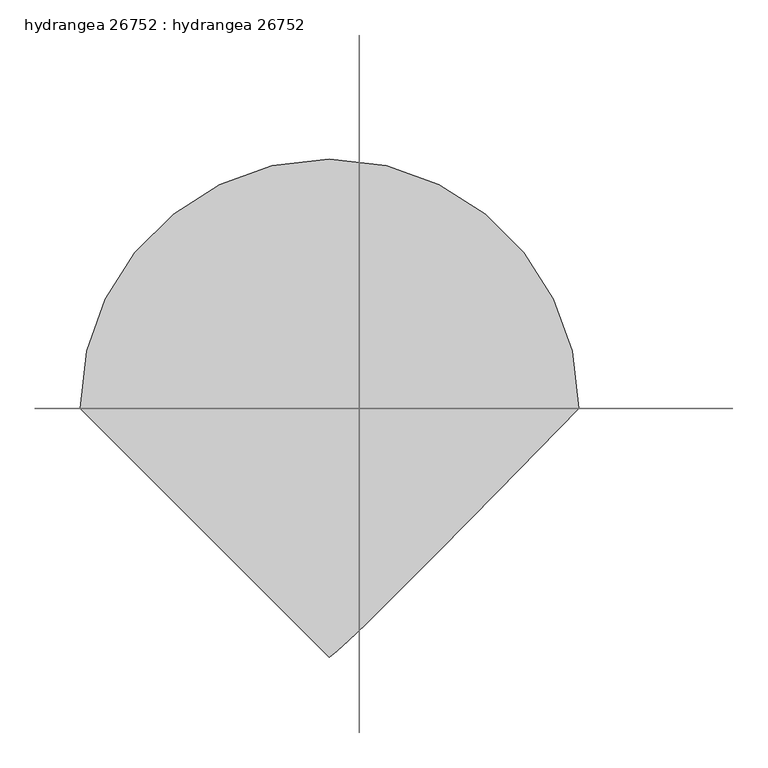
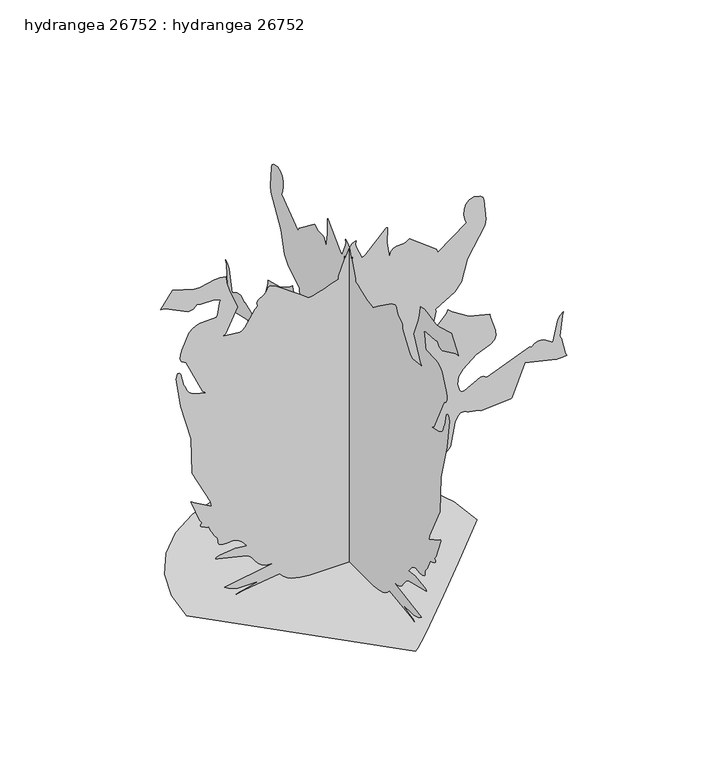
"""IFC4 building model written with IfcOpenShell, lengths in millimetres: proxy geometry, hydrangea 26752 : hydrangea 26752."""

from ifc_helpers import new_model, si_unit, origin, place, context, project, spatial, triangles, source, transform, mapped, element, save


def hydrangea_26752_hydrangea_26752_06a88d80(model_context):
    return source(origin(), model_context, "Body", "Tessellation", [
        triangles([(-464.7672343, 0.0, 3.02e-05), (-452.4787039, 106.4936905, 3.02e-05), (-417.4875984, 204.2914365, 3.02e-05), (-362.5905132, 290.5916013, 3.02e-05), (-290.5916013, 362.5905132, 3.02e-05), (-204.2911822, 417.4875984, 3.02e-05), (-106.4936905, 452.4787039, 3.02e-05), (2.03e-05, 464.7672343, 3.02e-05), (106.4939449, 452.4787039, 3.02e-05), (204.2914365, 417.4875984, 3.02e-05), (290.5916013, 362.5905132, 3.02e-05), (362.5905132, 290.5916013, 3.02e-05), (417.4875984, 204.2911822, 3.02e-05), (452.4787039, 106.4936905, 3.02e-05), (464.7672343, -4.06e-05, 3.02e-05), (313.7284884, -154.9290062, 3.02e-05), (201.7549816, -268.9964805, 3.02e-05), (122.337727, -349.0116546, 3.02e-05), (68.9646404, -401.7878663, 3.02e-05), (35.1246865, -434.1297149, 3.02e-05), (14.3067201, -452.8546257, 3.02e-05), (-6.09e-05, -464.7672343, 3.02e-05), (56.0289111, 377.7746518, 894.66276), (56.0289111, 434.8662978, 988.0256659), (56.0289111, 437.025323, 1007.8783058), (56.0289111, 431.6938534, 1074.0784075), (56.0289111, 427.5688871, 1084.5381615), (56.0289111, 420.2181004, 1091.4545998), (56.0289111, 399.2732306, 1096.0341894), (56.0289111, 384.089092, 1091.3859993), (56.0289111, 374.1170626, 1079.9991943), (56.0289111, 368.8109911, 1064.3553091), (56.0289111, 367.6197121, 1046.9435812), (56.0289111, 369.9971832, 1030.2455452), (56.0289111, 375.3946735, 1016.7479679), (56.0289111, 283.8809099, 949.5141357), (56.0289111, 278.4503729, 960.8348837), (56.0289111, 192.0161139, 1027.487138), (56.0289111, 183.512436, 1019.3997683), (56.0289111, 173.3158381, 1016.575304), (56.0289111, 151.4921339, 1016.077442), (56.0289111, 141.6905156, 1013.0776978), (56.0289111, 133.8441922, 1004.6956512), (56.0289111, 128.8665527, 988.2669302), (56.0289111, 120.2805761, 1038.0128763), (56.0289111, 121.9587531, 1087.6699471), (56.0289111, 121.3283319, 1088.8815737), (56.0289111, 120.3204537, 1089.2625824), (56.0289111, 119.0941387, 1088.975536), (56.0289111, 117.8101691, 1088.1856133), (56.0289111, 51.0174846, 1022.5290831), (56.0289111, 40.1538944, 1015.3484894), (56.0289111, 21.3923125, 1059.6105406), (56.0289111, 19.9031842, 1068.9729778), (56.0289111, 20.5441289, 1080.248089), (56.0289111, 9.1964113, 1074.4568727), (56.0289111, 0.5405762, 1063.7304199), (56.0289111, -13.2029357, 1031.7950146), (56.0289111, -15.0194446, 1031.1828426), (56.0289111, -16.1084712, 1040.5605406), (56.0289111, -15.8290449, 1030.10333), (56.0289111, -34.9326629, 980.1719301), (56.0289111, -34.6535171, 969.7147923), (56.0289111, -46.9016657, 965.6583538), (56.0289111, -59.853396, 960.979715), (56.0289111, -73.3885619, 956.0013124), (56.0289111, -87.3888065, 951.0482718), (56.0289111, -101.7342336, 946.4457911), (56.0289111, -116.3062366, 942.5138363), (56.0289111, -130.9854187, 939.5776056), (56.0289111, -158.8299491, 961.2921232), (56.0289111, -234.3038488, 1015.5618484), (56.0289111, -252.5433605, 1023.7431805), (56.0289111, -260.6957517, 1020.4259411), (56.0289111, -264.4829115, 1008.7952557), (56.0289111, -270.9573709, 1001.4368385), (56.0289111, -292.1841821, 987.7081707), (56.0289111, -295.084859, 980.1414814), (56.0289111, -293.5100641, 968.1907574), (56.0289111, -301.5567932, 960.9593674), (56.0289111, -333.5786213, 911.8103325), (56.0289111, -341.9555446, 903.575588), (56.0289111, -350.6474195, 900.6063652), (56.0289111, -405.2778059, 906.5576008), (56.0289111, -397.091387, 912.3182957), (56.0289111, -357.3022459, 989.5521715), (56.0289111, -383.3829941, 1051.2462982), (56.0289111, -392.869915, 1083.2706516), (56.0289111, -394.0713315, 1102.6610378), (56.0289111, -413.8020676, 1107.4693199), (56.0289111, -431.2518745, 1106.8977705), (56.0289111, -479.0928497, 1096.097703), (56.0289111, -496.5959965, 1097.2025774), (56.0289111, -565.8923844, 1117.6013323), (56.0289111, -605.1150993, 1065.3077946), (56.0289111, -590.4389603, 1063.2046526), (56.0289111, -515.963528, 1028.2542423), (56.0289111, -499.8980115, 1030.0398165), (56.0289111, -487.4520052, 1042.8973166), (56.0289111, -476.9008324, 1039.305748), (56.0289111, -431.2823596, 1037.8351255), (56.0289111, -421.2823886, 1035.6633831), (56.0289111, -412.7479531, 1030.7561245), (56.0289111, -416.4106656, 1023.8879391), (56.0289111, -422.1561361, 984.398489), (56.0289111, -425.8213557, 977.5278328), (56.0289111, -478.1860737, 974.7465345), (56.0289111, -490.5939646, 971.7493338), (56.0289111, -502.2144762, 965.7473019), (56.0289111, -512.7834532, 955.7015488), (56.0289111, -536.4029417, 906.3493286), (56.0289111, -540.7590348, 890.4260273), (56.0289111, -541.4473649, 876.4001392), (56.0289111, -536.9465132, 865.9378418), (56.0289111, -523.4413055, 857.3729576), (56.0289111, -470.3247439, 742.9737631), (56.0289111, -459.1462111, 734.3275612), (56.0289111, -495.4784048, 743.0092987), (56.0289111, -506.2683349, 747.8099504), (56.0289111, -515.3336246, 754.7263887), (56.0289111, -522.0366674, 764.454574), (56.0289111, -525.7400024, 777.6930828), (56.0289111, -531.1476665, 784.7339321), (56.0289111, -539.8243172, 825.0565435), (56.0289111, -543.8298866, 829.879941), (56.0289111, -550.6015663, 829.2856459), (56.0289111, -555.6434461, 813.3064613), (56.0289111, -540.8123746, 716.5628025), (56.0289111, -507.4392663, 594.6655191), (56.0289111, -503.093347, 475.8365441), (56.0289111, -444.0484045, 359.0446904), (56.0289111, -441.1045435, 344.0002235), (56.0289111, -497.2995872, 374.7622267), (56.0289111, -506.1286268, 381.752316), (56.0289111, -507.3122755, 379.8777938), (56.0289111, -479.3442879, 309.3622215), (56.0289111, -471.5769931, 298.1760402), (56.0289111, -476.8474926, 293.4109968), (56.0289111, -476.8347754, 288.7729441), (56.0289111, -473.0577893, 284.5159002), (56.0289111, -460.289201, 278.1963731), (56.0289111, -454.3303714, 276.6495199), (56.0289111, -450.6829196, 276.5250544), (56.0289111, -447.9727289, 270.8405358), (56.0289111, -445.4428688, 265.374445), (56.0289111, -442.9105016, 259.9769365), (56.0289111, -440.1901734, 254.4981467), (56.0289111, -437.1015175, 248.789756), (56.0289111, -433.4642395, 242.6990667), (56.0289111, -429.0903422, 236.0780501), (56.0289111, -423.9341526, 231.4173971), (56.0289111, -421.2519035, 226.5421133), (56.0289111, -420.2282742, 221.6594716), (56.0289111, -420.0530305, 216.9764544), (56.0289111, -419.910779, 212.7001166), (56.0289111, -418.9912857, 209.0374223), (56.0289111, -416.4817732, 206.1956808), (56.0289111, -404.3481751, 201.1304013), (56.0289111, -392.979138, 200.8065475), (56.0289111, -381.7802576, 202.325223), (56.0289111, -370.1622894, 202.7872406), (56.0289111, -357.5257424, 199.293722), (56.0289111, -343.2814084, 188.9454982), (56.0289111, -326.8374267, 168.843146), (56.0289111, -363.7335394, 174.8182537), (56.0289111, -415.2447847, 168.959745), (56.0289111, -424.7621907, 165.1799612), (56.0289111, -427.6882476, 161.3724901), (56.0289111, -422.6031655, 158.3819023), (56.0289111, -326.8374267, 135.2257031), (56.0289111, -316.3675352, 128.5444794), (56.0289111, -308.4071926, 119.1548454), (56.0289111, -301.2011826, 108.4708318), (56.0289111, -292.9842786, 97.9059425), (56.0289111, -281.9936886, 88.8741991), (56.0289111, -266.4742689, 82.7891145), (56.0289111, -244.6604659, 81.0642016), (56.0289111, -399.6745505, 54.9174055), (56.0289111, -387.1320385, 46.4490362), (56.0289111, -358.6535079, 37.4287247), (56.0289111, -291.3510571, 36.2410178), (56.0289111, -337.9144032, 23.9287606), (56.0289111, -349.4180614, 21.3156048), (56.0289111, -362.3212709, 18.4984871), (56.0289111, -355.630909, 19.454849), (56.0289111, -338.5316257, 22.4599004), (56.0289111, -314.6454383, 26.6484415), (56.0289111, -223.7308386, 37.9362155), (56.0289111, -211.5466986, 26.1533955), (56.0289111, -198.7755668, 17.3074794), (56.0289111, -185.515475, 10.9090339), (56.0289111, -171.8642371, 6.4684733), (56.0289111, -157.9193579, 3.4965937), (56.0289111, -143.7791599, 1.5035523), (56.0289111, -129.5409211, 0.0), (56.0289111, 156.3006158, 8.5e-06), (56.0289111, 151.6640893, 6.8894283), (56.0289111, 116.3057279, 38.9204668), (56.0289111, 111.4957199, 47.331436), (56.0289111, 111.590972, 55.6176853), (56.0289111, 119.3379828, 56.8782915), (56.0289111, 125.2241879, 59.5351333), (56.0289111, 130.2038621, 63.1188217), (56.0289111, 135.2315439, 67.1597133), (56.0289111, 141.2622714, 71.1881602), (56.0289111, 149.2498198, 74.7345099), (56.0289111, 160.1494906, 77.329128), (56.0289111, 168.9650681, 83.9521794), (56.0289111, 176.5355544, 87.5539036), (56.0289111, 196.7577757, 92.3169214), (56.0289111, 204.3280077, 95.9186456), (56.0289111, 213.1436033, 102.5419604), (56.0289111, 254.4092531, 106.5686224), (56.0289111, 265.3388912, 110.053257), (56.0289111, 275.7884532, 116.2788036), (56.0289111, 285.3972962, 126.1210626), (56.0289111, 270.7287694, 125.7187253), (56.0289111, 261.0386631, 129.5500684), (56.0289111, 244.0602664, 149.2523633), (56.0289111, 236.5088377, 152.8248832), (56.0289111, 225.0498715, 152.0344246), (56.0289111, 234.5898597, 172.6625532), (56.0289111, 246.2180017, 193.2690897), (56.0289111, 259.5756166, 213.3033683), (56.0289111, 323.1010995, 276.6977727), (56.0289111, 338.0566183, 354.6326777), (56.0289111, 345.6055398, 371.0131823), (56.0289111, 356.2354506, 380.7922002), (56.0289111, 370.7261358, 381.2874825), (56.0289111, 376.1719153, 376.5935466), (56.0289111, 382.951189, 373.9163844), (56.0289111, 414.431971, 368.0820022), (56.0289111, 421.1503109, 364.0103757), (56.0289111, 516.6848866, 372.087608), (56.0289111, 521.0689213, 374.2821688), (56.0289111, 561.6327971, 477.6729873), (56.0289111, 663.3141632, 454.759633), (56.0289111, 683.0017696, 454.2617709), (56.0289111, 696.6263014, 456.4588752), (56.0289111, 691.4650612, 464.9628256), (56.0289111, 679.3771362, 518.9251568), (56.0289111, 674.215896, 527.4291072), (56.0289111, 681.6479279, 594.9220805), (56.0289111, 685.4224068, 606.8042041), (56.0289111, 674.9575659, 597.7338638), (56.0289111, 667.4314991, 587.1039531), (56.0289111, 651.805418, 516.2225965), (56.0289111, 623.5224787, 533.9975653), (56.0289111, 613.96703, 536.3114865), (56.0289111, 604.0863831, 535.7831758), (56.0289111, 593.7181206, 531.7852003), (56.0289111, 582.7021142, 523.6927437), (56.0289111, 577.4646432, 527.2970295), (56.0289111, 440.4085831, 471.9960809), (56.0289111, 429.7609045, 477.805065), (56.0289111, 420.0225454, 479.0471403), (56.0289111, 367.9321567, 451.6074635), (56.0289111, 358.5290606, 450.3882792), (56.0289111, 353.3322121, 456.9262522), (56.0289111, 345.7960078, 481.3356634), (56.0289111, 350.0683125, 504.1753667), (56.0289111, 363.3880663, 525.0059266), (56.0289111, 406.1337856, 558.9200629), (56.0289111, 451.9579871, 579.6160017), (56.0289111, 465.1685543, 589.0190978), (56.0289111, 469.6389573, 603.0043633), (56.0289111, 467.9142806, 619.826774), (56.0289111, 451.0918336, 669.8597666), (56.0289111, 450.0987256, 680.5760456), (56.0289111, 383.0096157, 698.4017744), (56.0289111, 329.3240845, 731.7240864), (56.0289111, 316.5631265, 743.6087534), (56.0289111, 311.5136164, 731.6199503), (56.0289111, 280.6932047, 700.0375757), (56.0289111, 275.2499687, 690.0807707), (56.0289111, 272.6744173, 676.8397184), (56.0289111, 266.9721128, 689.0418806), (56.0289111, 265.8748323, 702.5623489), (56.0289111, 277.0838502, 752.2879475), (56.0289111, 276.1770741, 759.2500952), (56.0289111, 338.0413939, 796.367161), (56.0289111, 358.8363819, 823.4360029), (433.8020459, -5.25e-05, 894.66276), (490.8936919, -6.21e-05, 988.0256659), (493.0552242, -6.39e-05, 1007.8783058), (487.7237909, -6.93e-05, 1074.0784075), (483.5988247, -7.01e-05, 1084.5381615), (476.2454945, -7.04e-05, 1091.4545998), (455.3006247, -7.02e-05, 1096.0341894), (440.1164861, -6.93e-05, 1091.3859993), (430.1470001, -6.81e-05, 1079.9991943), (424.8383852, -6.66e-05, 1064.3553091), (423.6496496, -6.51e-05, 1046.9435812), (426.0270844, -6.37e-05, 1030.2455452), (431.4246111, -6.27e-05, 1016.7479679), (339.9082858, -5.44e-05, 949.5141357), (334.477767, -5.52e-05, 960.8348837), (248.0447615, -5.82e-05, 1027.487138), (239.541338, -5.73e-05, 1019.3997683), (229.3447583, -5.67e-05, 1016.575304), (207.5210541, -5.6e-05, 1016.077442), (197.7191814, -5.55e-05, 1013.0776978), (189.8731124, -5.45e-05, 1004.6956512), (184.8952004, -5.3e-05, 988.2669302), (176.3092419, -5.66e-05, 1038.0128763), (177.9874098, -6.11e-05, 1087.6699471), (177.3572339, -6.11e-05, 1088.8815737), (176.3491196, -6.1e-05, 1089.2625824), (175.1227954, -6.09e-05, 1088.975536), (173.8390802, -6.07e-05, 1088.1856133), (107.0464002, -5.35e-05, 1022.5290831), (96.182801, -5.27e-05, 1015.3484894), (77.4210737, -5.59e-05, 1059.6105406), (75.9321248, -5.66e-05, 1068.9729778), (76.5729696, -5.75e-05, 1080.248089), (65.2252475, -5.67e-05, 1074.4568727), (56.5694259, -5.55e-05, 1063.7304199), (42.8259742, -5.23e-05, 1031.7950146), (41.0093655, -5.23e-05, 1031.1828426), (39.9204648, -5.31e-05, 1040.5605406), (40.1998673, -5.22e-05, 1030.10333), (21.0960983, -4.75e-05, 980.1719301), (21.3753963, -4.66e-05, 969.7147923), (9.1270438, -4.59e-05, 965.6583538), (-3.8244574, -4.51e-05, 960.979715), (-17.3597019, -4.43e-05, 956.0013124), (-31.3598954, -4.34e-05, 951.0482718), (-45.7053225, -4.26e-05, 946.4457911), (-60.2773209, -4.18e-05, 942.5138363), (-74.9565076, -4.11e-05, 939.5776056), (-102.801038, -4.21e-05, 961.2921232), (-178.2749468, -4.45e-05, 1015.5618484), (-196.5144585, -4.46e-05, 1023.7431805), (-204.6668497, -4.41e-05, 1020.4259411), (-208.4534826, -4.3e-05, 1008.7952557), (-214.9284508, -4.22e-05, 1001.4368385), (-236.1547533, -4.05e-05, 987.7081707), (-239.055957, -3.97e-05, 980.1414814), (-237.481907, -3.88e-05, 968.1907574), (-245.5273643, -3.79e-05, 960.9593674), (-277.5486837, -3.28e-05, 911.8103325), (-285.9281505, -3.19e-05, 903.575588), (-294.6200436, -3.14e-05, 900.6063652), (-349.2479047, -3.02e-05, 906.5576008), (-341.0639929, -3.09e-05, 912.3182957), (-301.2723083, -3.86e-05, 989.5521715), (-327.3530565, -4.31e-05, 1051.2462982), (-336.8399775, -4.55e-05, 1083.2706516), (-338.0413939, -4.71e-05, 1102.6610378), (-357.77213, -4.69e-05, 1107.4693199), (-375.2244804, -4.63e-05, 1106.8977705), (-423.0654556, -4.4e-05, 1096.097703), (-440.5660953, -4.36e-05, 1097.2025774), (-509.8649903, -4.32e-05, 1117.6013323), (-549.0851618, -3.76e-05, 1065.3077946), (-534.4115662, -3.79e-05, 1063.2046526), (-459.9361339, -3.72e-05, 1028.2542423), (-443.8706174, -3.78e-05, 1030.0398165), (-431.4246111, -3.93e-05, 1042.8973166), (-420.8734383, -3.93e-05, 1039.305748), (-375.252422, -4.05e-05, 1037.8351255), (-365.252451, -4.06e-05, 1035.6633831), (-356.7180519, -4.05e-05, 1030.7561245), (-360.3832715, -3.98e-05, 1023.8879391), (-366.128742, -3.63e-05, 984.398489), (-369.7914182, -3.56e-05, 977.5278328), (-422.1586796, -3.38e-05, 974.7465345), (-434.5666068, -3.32e-05, 971.7493338), (-446.184575, -3.23e-05, 965.7473019), (-456.7535156, -3.12e-05, 955.7015488), (-480.3730042, -2.63e-05, 906.3493286), (-484.7290973, -2.48e-05, 890.4260273), (-485.4174637, -2.36e-05, 876.4001392), (-480.9165756, -2.29e-05, 865.9378418), (-467.4139114, -2.25e-05, 857.3729576), (-414.2948427, -1.45e-05, 742.9737631), (-403.118817, -1.41e-05, 734.3275612), (-439.4484673, -1.37e-05, 743.0092987), (-450.2383973, -1.38e-05, 747.8099504), (-459.303687, -1.42e-05, 754.7263887), (-466.0067662, -1.48e-05, 764.454574), (-469.7100649, -1.58e-05, 777.6930828), (-475.117729, -1.62e-05, 784.7339321), (-483.7943796, -1.93e-05, 825.0565435), (-487.7999854, -1.96e-05, 829.879941), (-494.5741722, -1.93e-05, 829.2856459), (-499.6160883, -1.78e-05, 813.3064613), (-484.782437, -1.01e-05, 716.5628025), (-451.4119085, -9e-07, 594.6655191), (-447.0659529, 9e-06, 475.8365441), (-388.0210467, 1.71e-05, 359.0446904), (-385.0746423, 1.83e-05, 344.0002235), (-441.2721931, 1.73e-05, 374.7622267), (-450.1012327, 1.7e-05, 381.752316), (-451.2848814, 1.73e-05, 379.8777938), (-423.3143867, 2.24e-05, 309.3622215), (-415.549599, 2.3e-05, 298.1760402), (-420.817555, 2.36e-05, 293.4109968), (-420.8048378, 2.39e-05, 288.7729441), (-417.0303952, 2.41e-05, 284.5159002), (-404.2592634, 2.42e-05, 278.1963731), (-398.3029773, 2.42e-05, 276.6495199), (-394.6555255, 2.42e-05, 276.5250544), (-391.9453348, 2.46e-05, 270.8405358), (-389.4129676, 2.5e-05, 265.374445), (-386.880564, 2.54e-05, 259.9769365), (-384.1602359, 2.58e-05, 254.4981467), (-381.0741234, 2.62e-05, 248.789756), (-377.4343019, 2.65e-05, 242.6990667), (-373.0604047, 2.7e-05, 236.0780501), (-367.9067585, 2.72e-05, 231.4173971), (-365.221966, 2.76e-05, 226.5421133), (-364.1983366, 2.8e-05, 221.6594716), (-364.0230929, 2.84e-05, 216.9764544), (-363.8808414, 2.87e-05, 212.7001166), (-362.9613482, 2.9e-05, 209.0374223), (-360.4543791, 2.92e-05, 206.1956808), (-348.320781, 2.92e-05, 201.1304013), (-336.9492004, 2.89e-05, 200.8065475), (-325.7528635, 2.84e-05, 202.325223), (-314.1323519, 2.81e-05, 202.7872406), (-301.4983665, 2.8e-05, 199.293722), (-287.2540325, 2.84e-05, 188.9454982), (-270.8075073, 2.96e-05, 168.843146), (-307.7036018, 3e-05, 174.8182537), (-359.2173906, 3.17e-05, 168.959745), (-368.7322532, 3.24e-05, 165.1799612), (-371.6583464, 3.32e-05, 161.3724901), (-366.5732643, 3.31e-05, 158.3819023), (-270.8075073, 3.24e-05, 135.2257031), (-260.3376158, 3.27e-05, 128.5444794), (-252.3792717, 3.32e-05, 119.1548454), (-245.1717719, 3.39e-05, 108.4708318), (-236.9543411, 3.46e-05, 97.9059425), (-225.9652771, 3.51e-05, 88.8741991), (-210.44484, 3.51e-05, 82.7891145), (-188.6315457, 3.46e-05, 81.0642016), (-343.6446493, 4.14e-05, 54.9174055), (-331.1021009, 4.15e-05, 46.4490362), (-302.6235885, 4.14e-05, 37.4287247), (-235.3221369, 3.98e-05, 36.2410178), (-281.887009, 4.21e-05, 23.9287856), (-293.3906855, 4.27e-05, 21.3156298), (-306.2913697, 4.33e-05, 18.498512), (-299.6009896, 4.31e-05, 19.454874), (-282.5016881, 4.23e-05, 22.4599277), (-258.6180442, 4.13e-05, 26.6484415), (-167.7021728, 3.76e-05, 37.9362155), (-155.5177784, 3.82e-05, 26.1533955), (-142.7466466, 3.86e-05, 17.3074794), (-129.4865639, 3.88e-05, 10.9090589), (-115.8353169, 3.87e-05, 6.4684733), (-101.8904468, 3.85e-05, 3.496619), (-87.7502488, 3.83e-05, 1.5035625), (-73.5122598, 3.8e-05, 9.2e-06), (212.3292817, 2.95e-05, 5.3e-06), (207.6930094, 2.9e-05, 6.8894283), (172.3346299, 2.74e-05, 38.9204668), (167.52464, 2.68e-05, 47.331436), (167.6196379, 2.61e-05, 55.6176853), (175.3668939, 2.58e-05, 56.8782915), (181.2528355, 2.54e-05, 59.5351333), (186.2325279, 2.49e-05, 63.1188217), (191.2602007, 2.44e-05, 67.1597133), (197.2911916, 2.39e-05, 71.1881602), (205.2787309, 2.34e-05, 74.7345099), (216.1781383, 2.29e-05, 77.329128), (224.9937339, 2.2e-05, 83.9521794), (232.5642021, 2.15e-05, 87.5539036), (252.7864416, 2.05e-05, 92.3169214), (260.3579453, 2e-05, 95.9186456), (269.1717423, 1.91e-05, 102.5419604), (310.4366472, 1.75e-05, 106.5686224), (321.3688288, 1.69e-05, 110.0530027), (331.8183726, 1.61e-05, 116.2788036), (341.4272338, 1.5e-05, 126.1210626), (326.7586887, 1.55e-05, 125.7187253), (317.0660391, 1.54e-05, 129.5500684), (300.0886597, 1.43e-05, 149.2523633), (292.5372311, 1.42e-05, 152.8248832), (281.0792822, 1.46e-05, 152.0344246), (290.6195429, 1.26e-05, 172.6625532), (302.2476667, 1.05e-05, 193.2690897), (315.6030107, 8.4e-06, 213.3033683), (379.1284936, 1.2e-06, 276.6977727), (394.0840124, -5.8e-06, 354.6326777), (401.6328976, -7.5e-06, 371.0131823), (412.2628083, -8.6e-06, 380.7922002), (426.7535299, -9.1e-06, 381.2874825), (432.1993094, -8.8e-06, 376.5935466), (438.9785831, -8.8e-06, 373.9163844), (470.4619085, -9.3e-06, 368.0820022), (477.1802121, -9.1e-06, 364.0103757), (572.7148241, -1.25e-05, 372.087608), (577.0988588, -1.3e-05, 374.2821688), (617.6601912, -2.29e-05, 477.6729873), (719.3415573, -2.4e-05, 454.759633), (739.0291637, -2.45e-05, 454.2617709), (752.6562389, -2.51e-05, 456.4588752), (747.4949987, -2.57e-05, 464.9628256), (735.4070738, -2.99e-05, 518.9251568), (730.2458336, -3.04e-05, 527.4291072), (737.6778654, -3.63e-05, 594.9220805), (741.4498009, -3.74e-05, 606.8042041), (730.9875034, -3.64e-05, 597.7338638), (723.4614367, -3.53e-05, 587.1039531), (707.8328121, -2.88e-05, 516.2225965), (679.5498728, -2.95e-05, 533.9975653), (669.9969675, -2.94e-05, 536.3114865), (660.1163206, -2.91e-05, 535.7831758), (649.7455147, -2.84e-05, 531.7852003), (638.729472, -2.74e-05, 523.6927437), (633.492001, -2.76e-05, 527.2970295), (496.4359772, -1.88e-05, 471.9960809), (485.7882986, -1.9e-05, 477.805065), (476.0524467, -1.88e-05, 479.0471403), (423.9620942, -1.49e-05, 451.6074635), (414.5564547, -1.45e-05, 450.3882792), (409.3621496, -1.49e-05, 456.9262522), (401.8259454, -1.72e-05, 481.3356634), (406.09825, -1.94e-05, 504.1753667), (419.4180038, -2.15e-05, 525.0059266), (462.1637232, -2.53e-05, 558.9200629), (507.9853812, -2.82e-05, 579.6160017), (521.1984919, -2.94e-05, 589.0190978), (525.6663514, -3.07e-05, 603.0043633), (523.9442182, -3.21e-05, 619.826774), (507.1192277, -3.58e-05, 669.8597666), (506.1286268, -3.66e-05, 680.5760456), (439.0370098, -3.62e-05, 698.4017744), (385.3514786, -3.74e-05, 731.7240864), (372.593064, -3.8e-05, 743.6087534), (367.5409741, -3.68e-05, 731.6199503), (336.7231241, -3.32e-05, 700.0375757), (331.2773809, -3.22e-05, 690.0807707), (328.7043549, -3.11e-05, 676.8397184), (323.0020503, -3.19e-05, 689.0418806), (321.9022264, -3.3e-05, 702.5623489), (333.1112443, -3.76e-05, 752.2879475), (332.2044683, -3.81e-05, 759.2500952), (394.0713315, -4.31e-05, 796.367161), (414.8663195, -4.6e-05, 823.4360029)], [[22, 21, 1], [21, 20, 1], [20, 19, 1], [19, 18, 1], [18, 17, 1], [1, 17, 2], [2, 17, 3], [3, 17, 4], [17, 16, 4], [4, 16, 5], [5, 16, 6], [6, 16, 7], [7, 16, 8], [8, 16, 9], [9, 16, 10], [10, 16, 11], [11, 16, 12], [16, 15, 12], [15, 14, 12], [14, 13, 12], [184, 183, 185], [60, 59, 61], [185, 183, 186], [183, 182, 186], [244, 243, 245], [178, 177, 179], [216, 215, 217], [196, 195, 197], [197, 195, 198], [186, 182, 187], [182, 181, 187], [187, 181, 188], [55, 54, 56], [95, 94, 96], [239, 238, 240], [198, 195, 199], [272, 271, 273], [168, 167, 169], [134, 133, 135], [215, 214, 217], [217, 214, 218], [179, 177, 180], [180, 177, 181], [167, 166, 169], [166, 165, 169], [165, 164, 169], [169, 164, 170], [38, 37, 39], [214, 213, 218], [96, 94, 97], [94, 93, 97], [97, 93, 98], [98, 93, 99], [93, 92, 99], [99, 92, 100], [100, 92, 101], [92, 91, 101], [91, 90, 101], [101, 90, 102], [90, 89, 102], [89, 88, 102], [88, 87, 102], [102, 87, 103], [199, 195, 200], [56, 54, 57], [54, 53, 57], [245, 243, 246], [243, 242, 246], [246, 242, 247], [242, 241, 247], [269, 268, 270], [103, 87, 104], [87, 86, 104], [104, 86, 105], [105, 86, 106], [86, 85, 106], [85, 84, 106], [135, 133, 136], [133, 132, 136], [136, 132, 137], [57, 53, 58], [126, 125, 127], [125, 124, 127], [124, 123, 127], [127, 123, 128], [123, 122, 128], [122, 121, 128], [121, 120, 128], [120, 119, 128], [53, 52, 58], [181, 177, 188], [119, 118, 128], [218, 213, 219], [219, 213, 220], [220, 213, 221], [213, 212, 221], [118, 117, 128], [170, 164, 171], [238, 237, 240], [240, 237, 241], [241, 237, 247], [247, 237, 248], [248, 237, 249], [249, 237, 250], [250, 237, 251], [251, 237, 252], [237, 236, 252], [252, 236, 253], [253, 236, 254], [236, 235, 254], [235, 234, 254], [234, 233, 254], [233, 232, 254], [254, 232, 255], [255, 232, 256], [256, 232, 257], [232, 231, 257], [231, 230, 257], [230, 229, 257], [257, 229, 258], [229, 228, 258], [106, 84, 107], [107, 84, 108], [108, 84, 109], [109, 84, 110], [110, 84, 111], [111, 84, 112], [112, 84, 113], [113, 84, 114], [114, 84, 115], [115, 84, 116], [116, 84, 117], [84, 83, 117], [271, 270, 273], [74, 73, 75], [73, 72, 75], [138, 137, 139], [139, 137, 140], [140, 137, 141], [137, 132, 141], [141, 132, 142], [142, 132, 143], [75, 72, 76], [228, 227, 258], [258, 227, 259], [128, 117, 129], [225, 224, 226], [47, 46, 48], [48, 46, 49], [49, 46, 50], [46, 45, 50], [50, 45, 51], [45, 44, 51], [51, 44, 52], [212, 211, 221], [211, 210, 221], [210, 209, 221], [83, 82, 117], [273, 270, 274], [274, 270, 275], [275, 270, 276], [265, 264, 266], [266, 264, 267], [267, 264, 268], [268, 264, 270], [264, 263, 270], [270, 263, 276], [263, 262, 276], [262, 261, 276], [58, 52, 59], [59, 52, 61], [61, 52, 62], [62, 52, 63], [52, 44, 63], [261, 260, 276], [72, 71, 76], [76, 71, 77], [77, 71, 78], [78, 71, 79], [79, 71, 80], [71, 70, 80], [80, 70, 81], [81, 70, 82], [82, 70, 117], [117, 70, 129], [129, 70, 130], [130, 70, 131], [70, 69, 131], [69, 68, 131], [68, 67, 131], [131, 67, 132], [67, 66, 132], [66, 65, 132], [65, 64, 132], [64, 63, 132], [63, 44, 132], [143, 132, 144], [132, 44, 144], [144, 44, 145], [145, 44, 146], [146, 44, 147], [147, 44, 148], [148, 44, 149], [149, 44, 150], [150, 44, 151], [151, 44, 152], [152, 44, 153], [153, 44, 154], [154, 44, 155], [155, 44, 156], [156, 44, 157], [157, 44, 158], [158, 44, 159], [159, 44, 160], [160, 44, 161], [161, 44, 162], [162, 44, 163], [163, 44, 164], [164, 44, 171], [171, 44, 172], [172, 44, 173], [173, 44, 174], [174, 44, 175], [175, 44, 176], [176, 44, 177], [177, 44, 188], [188, 44, 189], [189, 44, 190], [190, 44, 191], [191, 44, 192], [192, 44, 193], [193, 44, 194], [194, 44, 195], [195, 44, 200], [200, 44, 201], [201, 44, 202], [202, 44, 203], [203, 44, 204], [204, 44, 205], [205, 44, 206], [206, 44, 207], [207, 44, 208], [208, 44, 209], [209, 44, 221], [221, 44, 222], [222, 44, 223], [223, 44, 224], [224, 44, 226], [226, 44, 227], [227, 44, 259], [259, 44, 260], [44, 43, 260], [43, 42, 260], [30, 29, 31], [29, 28, 31], [31, 28, 32], [28, 27, 32], [27, 26, 32], [32, 26, 33], [33, 26, 34], [34, 26, 35], [26, 25, 35], [25, 24, 35], [24, 23, 35], [35, 23, 36], [23, 282, 36], [282, 281, 36], [281, 280, 36], [39, 37, 40], [36, 280, 37], [37, 280, 40], [40, 280, 41], [41, 280, 42], [280, 279, 42], [279, 278, 42], [278, 277, 42], [42, 277, 260], [260, 277, 276], [444, 443, 445], [320, 319, 321], [445, 443, 446], [443, 442, 446], [504, 503, 505], [438, 437, 439], [476, 475, 477], [456, 455, 457], [457, 455, 458], [446, 442, 447], [442, 441, 447], [447, 441, 448], [315, 314, 316], [355, 354, 356], [499, 498, 500], [458, 455, 459], [532, 531, 533], [428, 427, 429], [394, 393, 395], [475, 474, 477], [477, 474, 478], [439, 437, 440], [440, 437, 441], [427, 426, 429], [426, 425, 429], [425, 424, 429], [429, 424, 430], [298, 297, 299], [474, 473, 478], [356, 354, 357], [354, 353, 357], [357, 353, 358], [358, 353, 359], [353, 352, 359], [359, 352, 360], [360, 352, 361], [352, 351, 361], [351, 350, 361], [361, 350, 362], [350, 349, 362], [349, 348, 362], [348, 347, 362], [362, 347, 363], [459, 455, 460], [316, 314, 317], [314, 313, 317], [505, 503, 506], [503, 502, 506], [506, 502, 507], [502, 501, 507], [529, 528, 530], [363, 347, 364], [347, 346, 364], [364, 346, 365], [365, 346, 366], [346, 345, 366], [345, 344, 366], [395, 393, 396], [393, 392, 396], [396, 392, 397], [317, 313, 318], [386, 385, 387], [385, 384, 387], [384, 383, 387], [387, 383, 388], [383, 382, 388], [382, 381, 388], [381, 380, 388], [380, 379, 388], [313, 312, 318], [441, 437, 448], [379, 378, 388], [478, 473, 479], [479, 473, 480], [480, 473, 481], [473, 472, 481], [378, 377, 388], [430, 424, 431], [498, 497, 500], [500, 497, 501], [501, 497, 507], [507, 497, 508], [508, 497, 509], [509, 497, 510], [510, 497, 511], [511, 497, 512], [497, 496, 512], [512, 496, 513], [513, 496, 514], [496, 495, 514], [495, 494, 514], [494, 493, 514], [493, 492, 514], [514, 492, 515], [515, 492, 516], [516, 492, 517], [492, 491, 517], [491, 490, 517], [490, 489, 517], [517, 489, 518], [489, 488, 518], [366, 344, 367], [367, 344, 368], [368, 344, 369], [369, 344, 370], [370, 344, 371], [371, 344, 372], [372, 344, 373], [373, 344, 374], [374, 344, 375], [375, 344, 376], [376, 344, 377], [344, 343, 377], [531, 530, 533], [334, 333, 335], [333, 332, 335], [398, 397, 399], [399, 397, 400], [400, 397, 401], [397, 392, 401], [401, 392, 402], [402, 392, 403], [335, 332, 336], [488, 487, 518], [518, 487, 519], [388, 377, 389], [485, 484, 486], [307, 306, 308], [308, 306, 309], [309, 306, 310], [306, 305, 310], [310, 305, 311], [305, 304, 311], [311, 304, 312], [472, 471, 481], [471, 470, 481], [470, 469, 481], [343, 342, 377], [533, 530, 534], [534, 530, 535], [535, 530, 536], [525, 524, 526], [526, 524, 527], [527, 524, 528], [528, 524, 530], [524, 523, 530], [530, 523, 536], [523, 522, 536], [522, 521, 536], [318, 312, 319], [319, 312, 321], [321, 312, 322], [322, 312, 323], [312, 304, 323], [521, 520, 536], [332, 331, 336], [336, 331, 337], [337, 331, 338], [338, 331, 339], [339, 331, 340], [331, 330, 340], [340, 330, 341], [341, 330, 342], [342, 330, 377], [377, 330, 389], [389, 330, 390], [390, 330, 391], [330, 329, 391], [329, 328, 391], [328, 327, 391], [391, 327, 392], [327, 326, 392], [326, 325, 392], [325, 324, 392], [324, 323, 392], [323, 304, 392], [403, 392, 404], [392, 304, 404], [404, 304, 405], [405, 304, 406], [406, 304, 407], [407, 304, 408], [408, 304, 409], [409, 304, 410], [410, 304, 411], [411, 304, 412], [412, 304, 413], [413, 304, 414], [414, 304, 415], [415, 304, 416], [416, 304, 417], [417, 304, 418], [418, 304, 419], [419, 304, 420], [420, 304, 421], [421, 304, 422], [422, 304, 423], [423, 304, 424], [424, 304, 431], [431, 304, 432], [432, 304, 433], [433, 304, 434], [434, 304, 435], [435, 304, 436], [436, 304, 437], [437, 304, 448], [448, 304, 449], [449, 304, 450], [450, 304, 451], [451, 304, 452], [452, 304, 453], [453, 304, 454], [454, 304, 455], [455, 304, 460], [460, 304, 461], [461, 304, 462], [462, 304, 463], [463, 304, 464], [464, 304, 465], [465, 304, 466], [466, 304, 467], [467, 304, 468], [468, 304, 469], [469, 304, 481], [481, 304, 482], [482, 304, 483], [483, 304, 484], [484, 304, 486], [486, 304, 487], [487, 304, 519], [519, 304, 520], [304, 303, 520], [303, 302, 520], [290, 289, 291], [289, 288, 291], [291, 288, 292], [288, 287, 292], [287, 286, 292], [292, 286, 293], [293, 286, 294], [294, 286, 295], [286, 285, 295], [285, 284, 295], [284, 283, 295], [295, 283, 296], [283, 542, 296], [542, 541, 296], [541, 540, 296], [299, 297, 300], [296, 540, 297], [297, 540, 300], [300, 540, 301], [301, 540, 302], [540, 539, 302], [539, 538, 302], [538, 537, 302], [302, 537, 520], [520, 537, 536]], closed=False),
    ])


if __name__ == "__main__":
    model = new_model("IFC4")
    model_context = context("Model", 3, world=origin())
    ifc_project = project(units=[si_unit("LENGTHUNIT", "METRE", prefix="MILLI")], contexts=[model_context])
    site = spatial("IfcSite", under=ifc_project)
    building = spatial("IfcBuilding", under=site)
    placement = place(None, origin())
    hydrangea_26752_hydrangea_26752_shape = hydrangea_26752_hydrangea_26752_06a88d80(model_context)
    element("IfcBuildingElementProxy", 1, Name="hydrangea 26752 : hydrangea 26752", ObjectType="hydrangea 26752 : hydrangea 26752", at=placement, inside=building, context=model_context, shape_type="MappedRepresentation", body=[
        mapped(hydrangea_26752_hydrangea_26752_shape, transform((0.0, 0.0, 0.0), x_axis=(1.0, 0.0, 0.0), y_axis=(0.0, 1.0, 0.0), z_axis=(0.0, 0.0, 1.0))),
    ])
    save(model, "model.ifc")

# Revit data of these elements
# Type "hydrangea 26752 : hydrangea 26752"
#   built-in parameter 1005195 = "RPC-16-FW46-UP80-R12G-Q000-ST1L-LVER-AU"
#   Height = 0
